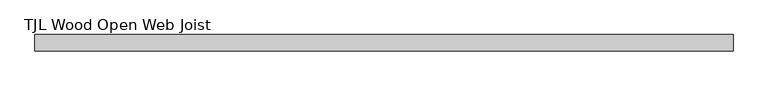
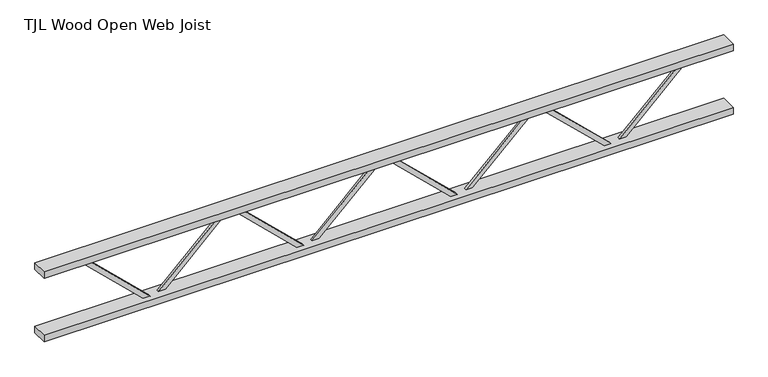
"""IFC4 building model written with IfcOpenShell, lengths in millimetres: beam geometry, TJL Wood Open Web Joist."""

from ifc_helpers import new_model, si_unit, frame, origin, place, context, project, spatial, polyline, outline, extrude, source, transform, mapped, element, save


def tjl_wood_open_web_joist_31b2a075(model_context):
    return source(origin(), model_context, "Body", "SweptSolid", [
        extrude(outline(polyline([(171.45, 842.9625), (196.85, 842.9625), (196.85, 825.1506163), (-171.45, 441.7693663), (-171.45, 396.08125), (-196.85, 396.08125), (-196.85, 451.9931337), (171.45, 835.3743837), (171.45, 842.9625)])), frame((0.0, 0.0, 0.0), z_axis=(0.0, 1.0, 0.0), x_axis=(0.0, 0.0, 1.0)), (0.0, 0.0, 1.0), 12.7),
        extrude(outline(polyline([(196.85, 0.0), (171.45, 0.0), (171.45, 7.5881163), (-196.85, 390.9693663), (-196.85, 446.88125), (-171.45, 446.88125), (-171.45, 401.1931337), (196.85, 17.8118837), (196.85, 0.0)])), frame((0.0, -12.7, 0.0), z_axis=(0.0, 1.0, 0.0), x_axis=(0.0, 0.0, 1.0)), (0.0, 0.0, 1.0), 12.7),
        extrude(outline(polyline([(171.45, 0.0), (196.85, 0.0), (196.85, -17.8118837), (-171.45, -401.1931337), (-171.45, -446.88125), (-196.85, -446.88125), (-196.85, -390.9693663), (171.45, -7.5881163), (171.45, 0.0)])), frame((0.0, 0.0, 0.0), z_axis=(0.0, 1.0, 0.0), x_axis=(0.0, 0.0, 1.0)), (0.0, 0.0, 1.0), 12.7),
        extrude(outline(polyline([(196.85, -842.9625), (171.45, -842.9625), (171.45, -835.3743837), (-196.85, -451.9931337), (-196.85, -396.08125), (-171.45, -396.08125), (-171.45, -441.7693663), (196.85, -825.1506163), (196.85, -842.9625)])), frame((0.0, -12.7, 0.0), z_axis=(0.0, 1.0, 0.0), x_axis=(0.0, 0.0, 1.0)), (0.0, 0.0, 1.0), 12.7),
        extrude(outline(polyline([(171.45, 1685.925), (196.85, 1685.925), (196.85, 1668.1131163), (-171.45, 1284.7318663), (-171.45, 1239.04375), (-196.85, 1239.04375), (-196.85, 1294.9556337), (171.45, 1678.3368837), (171.45, 1685.925)])), frame((0.0, 0.0, 0.0), z_axis=(0.0, 1.0, 0.0), x_axis=(0.0, 0.0, 1.0)), (0.0, 0.0, 1.0), 12.7),
        extrude(outline(polyline([(196.85, 842.9625), (171.45, 842.9625), (171.45, 850.5506163), (-196.85, 1233.9318663), (-196.85, 1289.84375), (-171.45, 1289.84375), (-171.45, 1244.1556337), (196.85, 860.7743837), (196.85, 842.9625)])), frame((0.0, -12.7, 0.0), z_axis=(0.0, 1.0, 0.0), x_axis=(0.0, 0.0, 1.0)), (0.0, 0.0, 1.0), 12.7),
        extrude(outline(polyline([(171.45, -842.9625), (196.85, -842.9625), (196.85, -860.7743837), (-171.45, -1244.1556337), (-171.45, -1289.84375), (-196.85, -1289.84375), (-196.85, -1233.9318663), (171.45, -850.5506163), (171.45, -842.9625)])), frame((0.0, 0.0, 0.0), z_axis=(0.0, 1.0, 0.0), x_axis=(0.0, 0.0, 1.0)), (0.0, 0.0, 1.0), 12.7),
        extrude(outline(polyline([(196.85, -1685.925), (171.45, -1685.925), (171.45, -1678.3368837), (-196.85, -1294.9556337), (-196.85, -1239.04375), (-171.45, -1239.04375), (-171.45, -1284.7318663), (196.85, -1668.1131163), (196.85, -1685.925)])), frame((0.0, -12.7, 0.0), z_axis=(0.0, 1.0, 0.0), x_axis=(0.0, 0.0, 1.0)), (0.0, 0.0, 1.0), 12.7),
        extrude(outline(polyline([(1889.125, 44.45), (1889.125, -44.45), (-1889.125, -44.45), (-1889.125, 44.45), (1889.125, 44.45)])), frame((0.0, 0.0, 165.1), z_axis=(0.0, 0.0, 1.0), x_axis=(1.0, 0.0, 0.0)), (0.0, 0.0, 1.0), 38.1),
        extrude(outline(polyline([(1889.125, 44.45), (1889.125, -44.45), (-1889.125, -44.45), (-1889.125, 44.45), (1889.125, 44.45)])), frame((0.0, 0.0, -203.2), z_axis=(0.0, 0.0, 1.0), x_axis=(1.0, 0.0, 0.0)), (0.0, 0.0, 1.0), 38.1),
    ])


if __name__ == "__main__":
    model = new_model("IFC4")
    model_context = context("Model", 3, world=origin())
    ifc_project = project(units=[si_unit("LENGTHUNIT", "METRE", prefix="MILLI")], contexts=[model_context])
    site = spatial("IfcSite", under=ifc_project)
    building = spatial("IfcBuilding", under=site)
    placement = place(None, origin())
    tjl_wood_open_web_joist_shape = tjl_wood_open_web_joist_31b2a075(model_context)
    element("IfcBeam", 1, ObjectType="TJL Wood Open Web Joist : 16\" PREENGINEERED FLOOR TRUSS", at=placement, inside=building, context=model_context, shape_type="MappedRepresentation", body=[
        mapped(tjl_wood_open_web_joist_shape, transform((0.0, 0.0, 0.0), x_axis=(1.0, 0.0, 0.0), y_axis=(0.0, 1.0, 0.0), z_axis=(0.0, 0.0, 1.0))),
    ])
    save(model, "model.ifc")

# Revit data of these elements
# Type "TJL Wood Open Web Joist : 16\" PREENGINEERED FLOOR TRUSS"
#   Web Thickness = 0' - 1"
#   Web Leg = 0' - 1"
#   Start Offset [instance default] = 0' - 0"
#   Top Chord Start Extension [instance default] = 0' - 0"
#   PanelArrayLength [instance default] = 22' - 8"
#   Depth = 1' - 4"
#   PanelWidth [instance default] = 2' - 6.22222"
#   Offset Length 2 [instance default] = 0' - 8"
#   Offset Length 1 [instance default] = 0' - 8"
#   End Panel [instance default] = 0' - 8"
#   End Offset [instance default] = 0' - 0"
#   Top Chord End Extension [instance default] = 0' - 0"
#   Chord Width = 0' - 3 1/2"
#   Chord Depth = 0' - 1 1/2"
#   Bottom Chord Start Extension [instance default] = 0' - 0"
#   Bottom Chord End Extension [instance default] = 0' - 0"
#   Length [instance default] = 24' - 0"
#   PanelArrayNum [instance default] = 9
#   Web Rendering Material = none
#   Structural Material = none
#   Assembly Code = ""
# Element 1 (IfcBeam, "TJL Wood Open Web Joist : 16\" PREENGINEERED FLOOR TRUSS")
#   PanelArrayLength = 11' - 0 3/4"
#   PanelWidth = 2' - 9 3/16"
#   PanelArrayNum = 4
